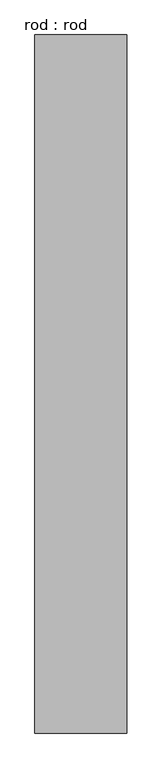
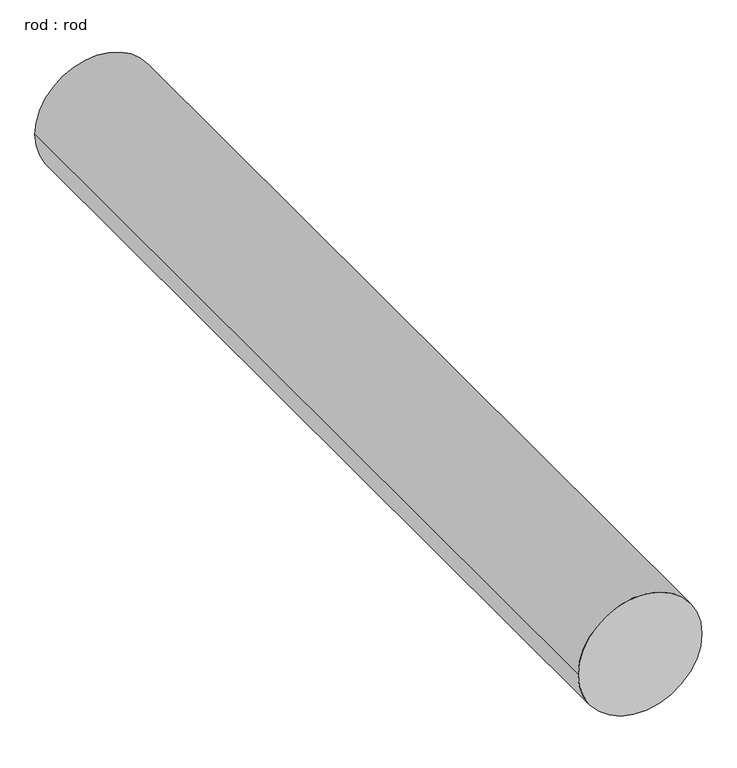
"""IFC4 building model written with IfcOpenShell, lengths in millimetres: proxy geometry, rod : rod."""

from ifc_helpers import new_model, si_unit, point, frame, frame_2d, origin, place, context, project, spatial, circle_curve, trimmed, segment, composite_curve, outline, extrude, source, transform, mapped, element, save


def rod_rod_a75019d7(model_context):
    return source(origin(), model_context, "Body", "SweptSolid", [
        extrude(outline(composite_curve([segment(trimmed(circle_curve(frame_2d((0.0108462, 0.0)), 200.0), [point((0.0108462, 200.0))], [point((0.0108462, -200.0))], False, "CARTESIAN"), True, "CONTINUOUS"), segment(trimmed(circle_curve(frame_2d((0.0108462, 0.0)), 200.0), [point((0.0108462, -200.0))], [point((0.0108462, 200.0))], False, "CARTESIAN"), True, "CONTINUOUS")], self_intersect=False)), frame((0.0, 2571.3000439, 0.0), z_axis=(0.0, 1.0, 0.0), x_axis=(0.0, 0.0, 1.0)), (0.0, 0.0, 1.0), 3042.8571429),
    ])


if __name__ == "__main__":
    model = new_model("IFC4")
    model_context = context("Model", 3, world=origin())
    ifc_project = project(units=[si_unit("LENGTHUNIT", "METRE", prefix="MILLI")], contexts=[model_context])
    site = spatial("IfcSite", under=ifc_project)
    building = spatial("IfcBuilding", under=site)
    placement = place(None, origin())
    rod_rod_shape = rod_rod_a75019d7(model_context)
    element("IfcBuildingElementProxy", 1, Name="rod : rod", ObjectType="rod : rod", at=placement, inside=building, context=model_context, shape_type="MappedRepresentation", body=[
        mapped(rod_rod_shape, transform((0.0, 0.0, 0.0), x_axis=(1.0, 0.0, 0.0), y_axis=(0.0, 1.0, 0.0), z_axis=(0.0, 0.0, 1.0))),
    ])
    save(model, "model.ifc")

# Revit data of these elements
# Type "rod : rod"
#   Default Elevation = 0
